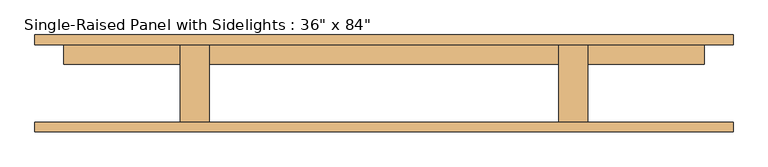
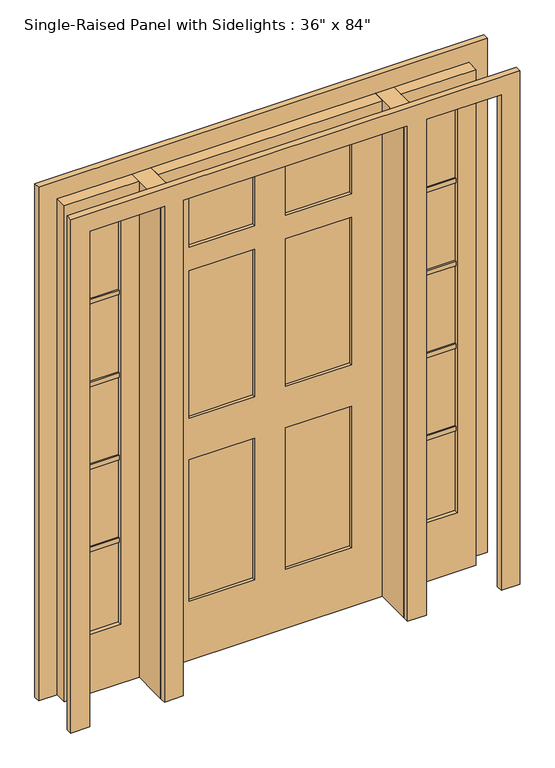
"""IFC4 building model written with IfcOpenShell, lengths in millimetres: door geometry."""

from ifc_helpers import new_model, si_unit, frame, origin, origin_with_axes, place, context, project, spatial, polyline, outline, extrude, source, transform, mapped, element, save


def door_4cad2e7a(model_context):
    return source(origin(), model_context, "Body", "SweptSolid", [
        extrude(outline(polyline([(762.0, 60.325), (609.6, 60.325), (609.6, 92.075), (762.0, 92.075), (762.0, 60.325)])), frame((0.0, 0.0, 600.075), z_axis=(0.0, 0.0, 1.0), x_axis=(1.0, 0.0, 0.0)), (0.0, 0.0, 1.0), 19.05),
        extrude(outline(polyline([(762.0, 60.325), (609.6, 60.325), (609.6, 92.075), (762.0, 92.075), (762.0, 60.325)])), frame((0.0, 0.0, 955.675), z_axis=(0.0, 0.0, 1.0), x_axis=(1.0, 0.0, 0.0)), (0.0, 0.0, 1.0), 19.05),
        extrude(outline(polyline([(762.0, 60.325), (609.6, 60.325), (609.6, 92.075), (762.0, 92.075), (762.0, 60.325)])), frame((0.0, 0.0, 1311.275), z_axis=(0.0, 0.0, 1.0), x_axis=(1.0, 0.0, 0.0)), (0.0, 0.0, 1.0), 19.05),
        extrude(outline(polyline([(762.0, 60.325), (609.6, 60.325), (609.6, 92.075), (762.0, 92.075), (762.0, 60.325)])), frame((0.0, 0.0, 1666.875), z_axis=(0.0, 0.0, 1.0), x_axis=(1.0, 0.0, 0.0)), (0.0, 0.0, 1.0), 19.05),
        extrude(outline(polyline([(-609.6, 60.325), (-762.0, 60.325), (-762.0, 92.075), (-609.6, 92.075), (-609.6, 60.325)])), frame((0.0, 0.0, 1666.875), z_axis=(0.0, 0.0, 1.0), x_axis=(1.0, 0.0, 0.0)), (0.0, 0.0, 1.0), 19.05),
        extrude(outline(polyline([(-609.6, 60.325), (-762.0, 60.325), (-762.0, 92.075), (-609.6, 92.075), (-609.6, 60.325)])), frame((0.0, 0.0, 1311.275), z_axis=(0.0, 0.0, 1.0), x_axis=(1.0, 0.0, 0.0)), (0.0, 0.0, 1.0), 19.05),
        extrude(outline(polyline([(-609.6, 60.325), (-762.0, 60.325), (-762.0, 92.075), (-609.6, 92.075), (-609.6, 60.325)])), frame((0.0, 0.0, 955.675), z_axis=(0.0, 0.0, 1.0), x_axis=(1.0, 0.0, 0.0)), (0.0, 0.0, 1.0), 19.05),
        extrude(outline(polyline([(-609.6, 60.325), (-762.0, 60.325), (-762.0, 92.075), (-609.6, 92.075), (-609.6, 60.325)])), frame((0.0, 0.0, 600.075), z_axis=(0.0, 0.0, 1.0), x_axis=(1.0, 0.0, 0.0)), (0.0, 0.0, 1.0), 19.05),
        extrude(outline(polyline([(762.0, 66.675), (609.6, 66.675), (609.6, 85.725), (762.0, 85.725), (762.0, 66.675)])), frame((0.0, 0.0, 254.0), z_axis=(0.0, 0.0, 1.0), x_axis=(1.0, 0.0, 0.0)), (0.0, 0.0, 1.0), 1778.0),
        extrude(outline(polyline([(-609.6, 66.675), (-762.0, 66.675), (-762.0, 85.725), (-609.6, 85.725), (-609.6, 66.675)])), frame((0.0, 0.0, 254.0), z_axis=(0.0, 0.0, 1.0), x_axis=(1.0, 0.0, 0.0)), (0.0, 0.0, 1.0), 1778.0),
        extrude(outline(polyline([(-457.2, -101.6), (-533.4, -101.6), (-533.4, 101.6), (-457.2, 101.6), (-457.2, -101.6)])), origin_with_axes(), (0.0, 0.0, 1.0), 2133.6),
        extrude(outline(polyline([(533.4, -101.6), (457.2, -101.6), (457.2, 101.6), (533.4, 101.6), (533.4, -101.6)])), origin_with_axes(), (0.0, 0.0, 1.0), 2133.6),
        extrude(outline(polyline([(2133.6, -533.4), (2133.6, -838.2), (0.0, -838.2), (0.0, -533.4), (2133.6, -533.4)]), holes=[polyline([(2032.0, -609.6), (254.0, -609.6), (254.0, -762.0), (2032.0, -762.0), (2032.0, -609.6)])]), frame((0.0, 50.8, 0.0), z_axis=(0.0, 1.0, 0.0), x_axis=(0.0, 0.0, 1.0)), (0.0, 0.0, 1.0), 50.8),
        extrude(outline(polyline([(0.0, 533.4), (0.0, 838.2), (2133.6, 838.2), (2133.6, 533.4), (0.0, 533.4)]), holes=[polyline([(2032.0, 762.0), (254.0, 762.0), (254.0, 609.6), (2032.0, 609.6), (2032.0, 762.0)])]), frame((0.0, 50.8, 0.0), z_axis=(0.0, 1.0, 0.0), x_axis=(0.0, 0.0, 1.0)), (0.0, 0.0, 1.0), 50.8),
        extrude(outline(polyline([(0.0, -914.4), (0.0, -838.2), (2133.6, -838.2), (2133.6, -533.4), (0.0, -533.4), (0.0, -457.2), (2133.6, -457.2), (2133.6, 457.2), (0.0, 457.2), (0.0, 533.4), (2133.6, 533.4), (2133.6, 838.2), (0.0, 838.2), (0.0, 914.4), (2209.8, 914.4), (2209.8, -914.4), (0.0, -914.4)])), frame((0.0, -127.0, 0.0), z_axis=(0.0, 1.0, 0.0), x_axis=(0.0, 0.0, 1.0)), (0.0, 0.0, 1.0), 25.4),
        extrude(outline(polyline([(0.0, 914.4), (2209.8, 914.4), (2209.8, -914.4), (0.0, -914.4), (0.0, -838.2), (2133.6, -838.2), (2133.6, -533.4), (0.0, -533.4), (0.0, -457.2), (2133.6, -457.2), (2133.6, 457.2), (0.0, 457.2), (0.0, 533.4), (2133.6, 533.4), (2133.6, 838.2), (0.0, 838.2), (0.0, 914.4)])), frame((0.0, 101.6, 0.0), z_axis=(0.0, 1.0, 0.0), x_axis=(0.0, 0.0, 1.0)), (0.0, 0.0, 1.0), 25.4),
        extrude(outline(polyline([(-63.5, 63.5), (-330.2, 63.5), (-330.2, 88.9), (-63.5, 88.9), (-63.5, 63.5)])), frame((0.0, 0.0, 1778.0), z_axis=(0.0, 0.0, 1.0), x_axis=(1.0, 0.0, 0.0)), (0.0, 0.0, 1.0), 254.0),
        extrude(outline(polyline([(330.2, 63.5), (63.5, 63.5), (63.5, 88.9), (330.2, 88.9), (330.2, 63.5)])), frame((0.0, 0.0, 1778.0), z_axis=(0.0, 0.0, 1.0), x_axis=(1.0, 0.0, 0.0)), (0.0, 0.0, 1.0), 254.0),
        extrude(outline(polyline([(-63.5, 63.5), (-330.2, 63.5), (-330.2, 88.9), (-63.5, 88.9), (-63.5, 63.5)])), frame((0.0, 0.0, 1041.4), z_axis=(0.0, 0.0, 1.0), x_axis=(1.0, 0.0, 0.0)), (0.0, 0.0, 1.0), 635.0),
        extrude(outline(polyline([(330.2, 63.5), (63.5, 63.5), (63.5, 88.9), (330.2, 88.9), (330.2, 63.5)])), frame((0.0, 0.0, 1041.4), z_axis=(0.0, 0.0, 1.0), x_axis=(1.0, 0.0, 0.0)), (0.0, 0.0, 1.0), 635.0),
        extrude(outline(polyline([(-63.5, 63.5), (-330.2, 63.5), (-330.2, 88.9), (-63.5, 88.9), (-63.5, 63.5)])), frame((0.0, 0.0, 254.0), z_axis=(0.0, 0.0, 1.0), x_axis=(1.0, 0.0, 0.0)), (0.0, 0.0, 1.0), 609.6),
        extrude(outline(polyline([(330.2, 63.5), (63.5, 63.5), (63.5, 88.9), (330.2, 88.9), (330.2, 63.5)])), frame((0.0, 0.0, 254.0), z_axis=(0.0, 0.0, 1.0), x_axis=(1.0, 0.0, 0.0)), (0.0, 0.0, 1.0), 609.6),
        extrude(outline(polyline([(2133.6, 457.2), (2133.6, -457.2), (0.0, -457.2), (0.0, 457.2), (2133.6, 457.2)]), holes=[polyline([(2032.0, -63.5), (1778.0, -63.5), (1778.0, -330.2), (2032.0, -330.2), (2032.0, -63.5)]), polyline([(2032.0, 330.2), (1778.0, 330.2), (1778.0, 63.5), (2032.0, 63.5), (2032.0, 330.2)]), polyline([(1676.4, -63.5), (1041.4, -63.5), (1041.4, -330.2), (1676.4, -330.2), (1676.4, -63.5)]), polyline([(1676.4, 330.2), (1041.4, 330.2), (1041.4, 63.5), (1676.4, 63.5), (1676.4, 330.2)]), polyline([(863.6, -63.5), (254.0, -63.5), (254.0, -330.2), (863.6, -330.2), (863.6, -63.5)]), polyline([(863.6, 330.2), (254.0, 330.2), (254.0, 63.5), (863.6, 63.5), (863.6, 330.2)])]), frame((0.0, 50.8, 0.0), z_axis=(0.0, 1.0, 0.0), x_axis=(0.0, 0.0, 1.0)), (0.0, 0.0, 1.0), 50.8),
    ])


if __name__ == "__main__":
    model = new_model("IFC4")
    model_context = context("Model", 3, world=origin())
    ifc_project = project(units=[si_unit("LENGTHUNIT", "METRE", prefix="MILLI")], contexts=[model_context])
    site = spatial("IfcSite", under=ifc_project)
    building = spatial("IfcBuilding", under=site)
    placement = place(None, origin())
    door_shape = door_4cad2e7a(model_context)
    element("IfcDoor", 1, ObjectType="Single-Raised Panel with Sidelights : 36\" x 84\"", at=placement, inside=building, context=model_context, shape_type="MappedRepresentation", body=[
        mapped(door_shape, transform((0.0, 0.0, 0.0), x_axis=(1.0, 0.0, 0.0), y_axis=(0.0, 1.0, 0.0), z_axis=(0.0, 0.0, 1.0))),
    ])
    save(model, "model.ifc")

# Revit data of these elements
# Type "Single-Raised Panel with Sidelights : 36\" x 84\""
#   Type Mark = "41"
#   Assembly Code = "C1020"
#   Thickness = 0' - 2"
#   Height = 7' - 0"
#   Rail Width - Base = 0' - 10"
#   Rail Width - Center = 0' - 7"
#   Rail Width - Top = 0' - 4"
#   Sidelight Width = 1' - 0"
#   Stile Width = 0' - 5"
#   Trim Projection Ext = 0' - 1"
#   Trim Projection Int = 0' - 1"
#   Trim Width = 0' - 3"
#   Width = 3' - 0"
#   Define Thermal Properties by = 0
#   Function = 1
#   Door Material = Door - Panel
#   Frame Material = Door - Frame
#   Wall Closure = (empty or 0)
# Element 1 (IfcDoor, "Single-Raised Panel with Sidelights : 36\" x 84\"")
#   Materials on its faces: "Door - Panel", "Door - Frame", "Glass"
# Materials
#   "Door - Panel": class "Wood", colour RGB 227 170 128, transparency 0, Cost = 0
#   "Door - Frame": class "Miscellaneous", colour RGB 153 76 43, transparency 0, Cost = 0
#   "Glass": class "Glass", colour RGB 236 240 239, transparency 0.5, Description = "Soda Lime Glass", Cost = 0
